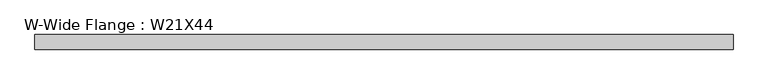
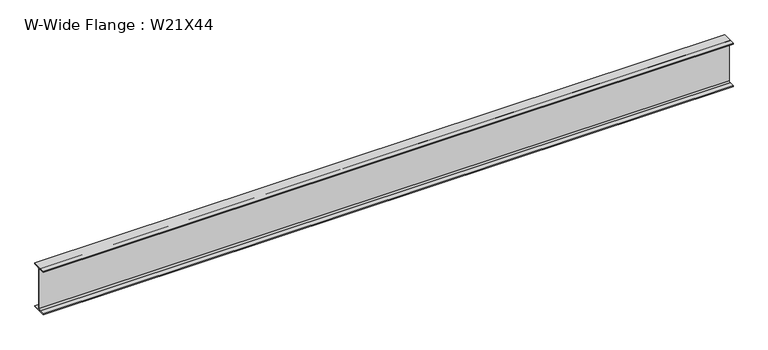
"""IFC4 building model written with IfcOpenShell, lengths in millimetres: beam geometry, W-Wide Flange : W21X44."""

from ifc_helpers import new_model, si_unit, point, frame, frame_2d, origin, place, context, project, spatial, polyline, circle_curve, trimmed, segment, composite_curve, outline, extrude, source, transform, mapped, element, save


def w_wide_flange_w21x44_aeefe74e(model_context):
    return source(origin(), model_context, "Body", "SweptSolid", [
        extrude(outline(composite_curve([segment(polyline([(82.55, -251.46), (82.55, -262.89), (-82.55, -262.89), (-82.55, -251.46), (-21.59, -251.46)]), True, "CONTINUOUS"), segment(trimmed(circle_curve(frame_2d((-21.59, -234.315)), 17.145), [point((-21.59, -251.46))], [point((-4.445, -234.315))], True, "CARTESIAN"), True, "CONTINUOUS"), segment(polyline([(-4.445, -234.315), (-4.445, 234.315)]), True, "CONTINUOUS"), segment(trimmed(circle_curve(frame_2d((-21.59, 234.315)), 17.145), [point((-4.445, 234.315))], [point((-21.59, 251.46))], True, "CARTESIAN"), True, "CONTINUOUS"), segment(polyline([(-21.59, 251.46), (-82.55, 251.46), (-82.55, 262.89), (82.55, 262.89), (82.55, 251.46), (21.59, 251.46)]), True, "CONTINUOUS"), segment(trimmed(circle_curve(frame_2d((21.59, 234.315)), 17.145), [point((21.59, 251.46))], [point((4.445, 234.315))], True, "CARTESIAN"), True, "CONTINUOUS"), segment(polyline([(4.445, 234.315), (4.445, -234.315)]), True, "CONTINUOUS"), segment(trimmed(circle_curve(frame_2d((21.59, -234.315)), 17.145), [point((4.445, -234.315))], [point((21.59, -251.46))], True, "CARTESIAN"), True, "CONTINUOUS"), segment(polyline([(21.59, -251.46), (82.55, -251.46)]), True, "CONTINUOUS")], self_intersect=False)), frame((-3903.7559594, 0.0, 0.0), z_axis=(1.0, 0.0, 0.0), x_axis=(0.0, 1.0, 0.0)), (0.0, 0.0, 1.0), 7868.0918251),
    ])


if __name__ == "__main__":
    model = new_model("IFC4")
    model_context = context("Model", 3, world=origin())
    ifc_project = project(units=[si_unit("LENGTHUNIT", "METRE", prefix="MILLI")], contexts=[model_context])
    site = spatial("IfcSite", under=ifc_project)
    building = spatial("IfcBuilding", under=site)
    placement = place(None, origin())
    w_wide_flange_w21x44_shape = w_wide_flange_w21x44_aeefe74e(model_context)
    element("IfcBeam", 1, ObjectType="W-Wide Flange : W21X44", at=placement, inside=building, context=model_context, shape_type="MappedRepresentation", body=[
        mapped(w_wide_flange_w21x44_shape, transform((0.0, 0.0, 0.0), x_axis=(1.0, 0.0, 0.0), y_axis=(0.0, 1.0, 0.0), z_axis=(0.0, 0.0, 1.0))),
    ])
    save(model, "model.ifc")

# Revit data of these elements
# Type "W-Wide Flange : W21X44"
#   Assembly Code = "B10"
#   W = 44
#   Length [instance default] = 1524 mm
#   bf = 165.1 mm
#   d = 525.78 mm
#   k = 28.575 mm
#   k2 = 17.145 mm
#   tf = 11.43 mm
#   tw = 8.89 mm
#   A = 0.00838708 m²
#   Structural Material [instance default] = Steel ASTM A992
# Element 1 (IfcBeam, "W-Wide Flange : W21X44")
#   Structural Material = Aluminum, Anodized Red
#   Materials on its faces: "Aluminum, Anodized Red"
# Materials
#   "Steel ASTM A992": class "Metal", colour RGB 128 0 0, transparency 0, Description = "Structural steel 50ksi", Cost = 0
#   "Aluminum, Anodized Red": class "Metal", colour RGB 120 120 120, transparency 0, Description = "Anodized aluminum, red", Cost = 0
